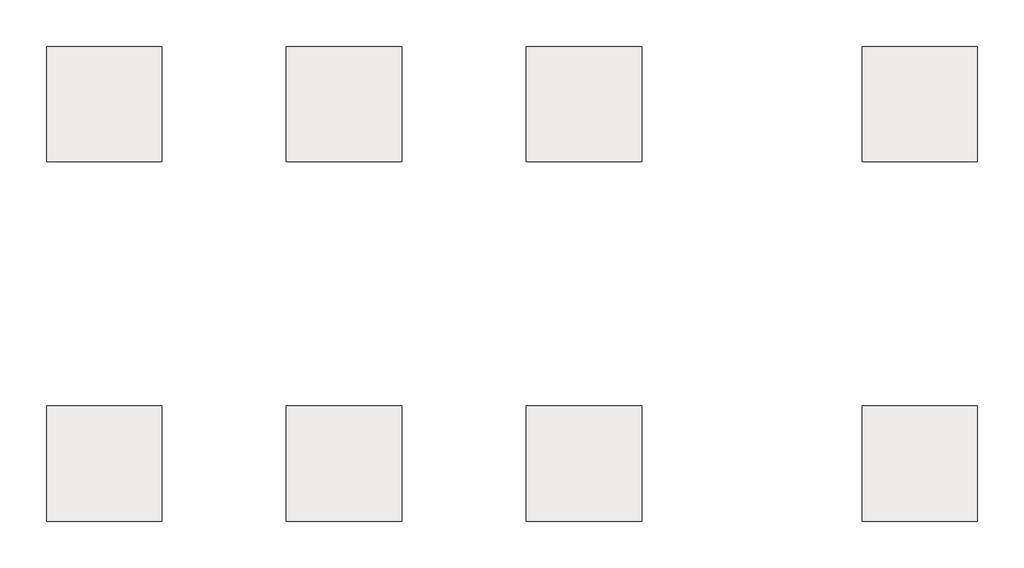
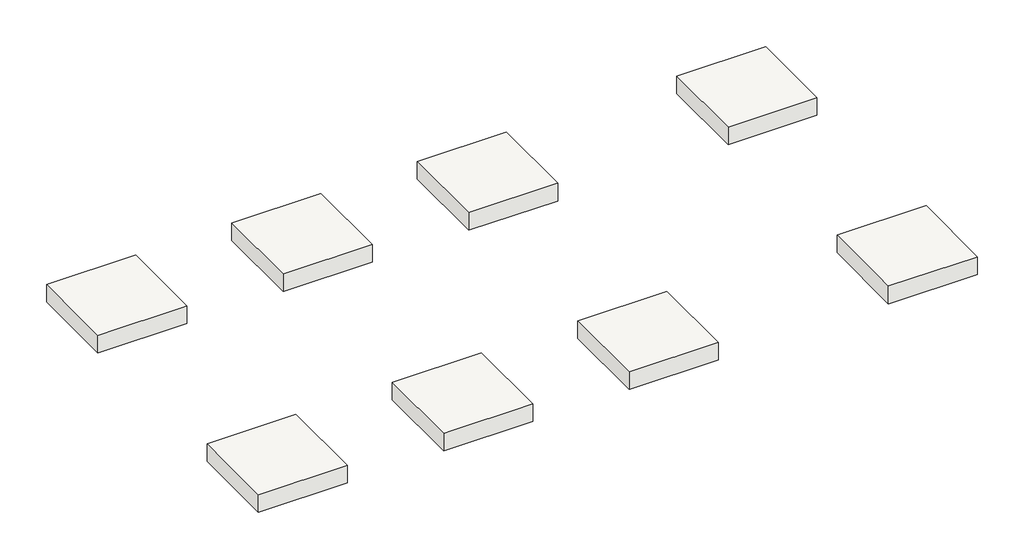
# Not in any storey: 8 slabs.
"""IFC4 building model written with IfcOpenShell, lengths in millimetres."""

import ifcopenshell
import ifcopenshell.guid

model = None  # the IFC model being written
_history = None  # IfcOwnerHistory: only IFC2X3 demands one
_inside = {}  # id of a spatial element -> (the spatial element, [elements in it])
_under = {}  # id of a project, library or spatial element -> (it, [spatial elements below it])
_declared = {}  # id of a project -> (the project, [libraries it declares])
_typed = {}  # id of a type object -> (the type object, [elements of that type])
_made_of = {}  # id of a material, layer set ... -> (it, [elements and type objects made of it])


def new_model(schema):
    """Start an empty IFC model of exactly this schema.

    Asked for "IFC4X3", IfcOpenShell would pick the latest addendum, in which some entities
    have other attributes; the version numbers below select the first issue.
    IFC2X3 requires an IfcOwnerHistory on every rooted entity: one is made here for all.
    """
    global model, _history
    if schema == "IFC4X3":
        model = ifcopenshell.file(schema_version=(4, 3, 0, 0))
    else:
        model = ifcopenshell.file(schema=schema)
    _inside.clear()
    _under.clear()
    _declared.clear()
    _typed.clear()
    _made_of.clear()
    _history = None
    if model.schema == "IFC2X3":
        org = make("IfcOrganization", Name="unknown")
        user = make(
            "IfcPersonAndOrganization",
            ThePerson=make("IfcPerson", FamilyName="unknown"),
            TheOrganization=org,
        )
        app = make(
            "IfcApplication",
            ApplicationDeveloper=org,
            Version="unknown",
            ApplicationFullName="unknown",
            ApplicationIdentifier="unknown",
        )
        _history = make(
            "IfcOwnerHistory",
            OwningUser=user,
            OwningApplication=app,
            ChangeAction="ADDED",
            CreationDate=0,
        )
    return model


def make(cls, **values):
    """One entity of the class cls with the attributes given. An attribute that is None is left unset."""
    return model.create_entity(
        cls, **{name: value for name, value in values.items() if value is not None}
    )


def rooted(cls, **values):
    """An entity with a GlobalId (a new one), such as an element, a storey or a relation."""
    return make(cls, GlobalId=ifcopenshell.guid.new(), OwnerHistory=_history, **values)


def si_unit(unit_type, name, prefix=None):
    """IfcSIUnit, for example si_unit("LENGTHUNIT", "METRE", prefix="MILLI")."""
    return make("IfcSIUnit", UnitType=unit_type, Prefix=prefix, Name=name)


def assignment(units):
    """IfcUnitAssignment: the units of a project."""
    return None if units is None else make("IfcUnitAssignment", Units=units)


def point(xyz):
    """IfcCartesianPoint."""
    return None if xyz is None else make("IfcCartesianPoint", Coordinates=xyz)


def direction(xyz):
    """IfcDirection."""
    return None if xyz is None else make("IfcDirection", DirectionRatios=xyz)


def frame(location, z_axis=None, x_axis=None):
    """IfcAxis2Placement3D, a coordinate frame: its origin and axes. An axis left out is left unset."""
    return make(
        "IfcAxis2Placement3D",
        Location=point(location),
        Axis=direction(z_axis),
        RefDirection=direction(x_axis),
    )


def origin():
    """The frame at (0, 0, 0) with its axes left unset."""
    return frame((0.0, 0.0, 0.0))


def place(relative_to, where):
    """IfcLocalPlacement: puts the frame where relative to a parent placement (None: the world)."""
    return make(
        "IfcLocalPlacement", PlacementRelTo=relative_to, RelativePlacement=where
    )


def context(
    kind, dimensions, precision=None, world=None, true_north=None, identifier=None
):
    """IfcGeometricRepresentationContext, for example the 3D "Model" context."""
    return make(
        "IfcGeometricRepresentationContext",
        ContextIdentifier=identifier,
        ContextType=kind,
        CoordinateSpaceDimension=dimensions,
        Precision=precision,
        WorldCoordinateSystem=world,
        TrueNorth=true_north,
    )


def project(units=None, contexts=None):
    """IfcProject with its units and contexts."""
    return rooted(
        "IfcProject",
        Name="project",
        RepresentationContexts=contexts,
        UnitsInContext=assignment(units),
    )


def spatial(cls, under=None, at=None, **own):
    """A site, building, storey or space (cls), placed at a placement, below another one or the project."""
    s = rooted(cls, ObjectPlacement=at, **own)
    if under is not None:
        _under.setdefault(under.id(), (under, []))[1].append(s)
    return s


def polyline(points):
    """IfcPolyline through the points."""
    return make("IfcPolyline", Points=[point(p) for p in points])


def outline(outer, holes=None, kind="AREA"):
    """IfcArbitraryClosedProfileDef: a profile drawn as a closed curve; with holes, ...WithVoids."""
    if holes is None:
        return make("IfcArbitraryClosedProfileDef", ProfileType=kind, OuterCurve=outer)
    return make(
        "IfcArbitraryProfileDefWithVoids",
        ProfileType=kind,
        OuterCurve=outer,
        InnerCurves=holes,
    )


def extrude(swept, where, along, depth):
    """IfcExtrudedAreaSolid: the profile swept, set in the frame where, extruded along a direction by depth."""
    return make(
        "IfcExtrudedAreaSolid",
        SweptArea=swept,
        Position=where,
        ExtrudedDirection=direction(along),
        Depth=depth,
    )


def shape(context_of_items, identifier, shape_type, items):
    """IfcShapeRepresentation: the items that make up one representation, for example the "Body"."""
    return make(
        "IfcShapeRepresentation",
        ContextOfItems=context_of_items,
        RepresentationIdentifier=identifier,
        RepresentationType=shape_type,
        Items=items,
    )


def source(mapping_origin, context_of_items, identifier, shape_type, items):
    """IfcRepresentationMap: a shape defined once, which mapped items show again and again."""
    return make(
        "IfcRepresentationMap",
        MappingOrigin=mapping_origin,
        MappedRepresentation=shape(context_of_items, identifier, shape_type, items),
    )


def transform(
    local_origin,
    x_axis=None,
    y_axis=None,
    z_axis=None,
    scale=None,
    scale2=None,
    scale3=None,
    uniform=True,
):
    """IfcCartesianTransformationOperator3D, or its non-uniform kind. x_axis, y_axis, z_axis: its Axis1, 2, 3."""
    if uniform:
        return make(
            "IfcCartesianTransformationOperator3D",
            Axis1=direction(x_axis),
            Axis2=direction(y_axis),
            LocalOrigin=point(local_origin),
            Scale=scale,
            Axis3=direction(z_axis),
        )
    return make(
        "IfcCartesianTransformationOperator3DnonUniform",
        Axis1=direction(x_axis),
        Axis2=direction(y_axis),
        LocalOrigin=point(local_origin),
        Scale=scale,
        Axis3=direction(z_axis),
        Scale2=scale2,
        Scale3=scale3,
    )


def mapped(mapping_source, mapping_target):
    """IfcMappedItem: shows the shape of a source again, moved by a transform."""
    return make(
        "IfcMappedItem", MappingSource=mapping_source, MappingTarget=mapping_target
    )


def made_of(thing, what):
    """Note that an element or type object is made of a material, layer set ...; save() writes the relation."""
    if what is not None:
        _made_of.setdefault(what.id(), (what, []))[1].append(thing)
    return thing


def element(
    cls,
    number,
    at=None,
    inside=None,
    cuts=None,
    type_object=None,
    material=None,
    context=None,
    identifier="Body",
    shape_type=None,
    held_by="IfcProductDefinitionShape",
    body=None,
    shapes=None,
    **own,
):
    """One element of the class cls, such as IfcWall. Its Tag is "e" and its number.

    at: its placement. inside: the storey or other place that contains it. cuts: it is an
    opening in that element (IfcRelVoidsElement). A single representation is given by context,
    identifier, shape_type and body (its items); several are given by shapes. held_by: the class
    of the entity that holds the representations. save() writes the other relations.
    """
    e = rooted(cls, Tag="e%d" % number, ObjectPlacement=at, **own)
    if body is not None:
        shapes = [shape(context, identifier, shape_type, body)]
    if shapes is not None:
        e.Representation = make(held_by, Representations=shapes)
    if inside is not None:
        _inside.setdefault(inside.id(), (inside, []))[1].append(e)
    if cuts is not None:
        rooted(
            "IfcRelVoidsElement", RelatingBuildingElement=cuts, RelatedOpeningElement=e
        )
    if type_object is not None:
        _typed.setdefault(type_object.id(), (type_object, []))[1].append(e)
    return made_of(e, material)


def aggregate(whole, parts):
    """IfcRelAggregates: a whole, such as a stair, and the parts it consists of."""
    return rooted("IfcRelAggregates", RelatingObject=whole, RelatedObjects=parts)


def save(model, path):
    """Write the relations noted so far, then the file.

    IfcRelAggregates (storeys below a building ...), IfcRelContainedInSpatialStructure (elements
    in a storey), IfcRelDefinesByType, IfcRelAssociatesMaterial and IfcRelDeclares: one each for
    every whole, place, type object, material and project.
    """
    for whole, parts in _under.values():
        aggregate(whole, parts)
    for where, things in _inside.values():
        rooted(
            "IfcRelContainedInSpatialStructure",
            RelatedElements=things,
            RelatingStructure=where,
        )
    for kind, things in _typed.values():
        rooted("IfcRelDefinesByType", RelatedObjects=things, RelatingType=kind)
    for what, things in _made_of.values():
        rooted("IfcRelAssociatesMaterial", RelatedObjects=things, RelatingMaterial=what)
    for by, libraries in _declared.values():
        rooted("IfcRelDeclares", RelatingContext=by, RelatedDefinitions=libraries)
    model.write(path)


def ft211_footing_rectangular_r0_ft211_footing_rectangular_5fe39465(model_context):
    return source(origin(), model_context, "Body", "SweptSolid", [
        extrude(outline(polyline([(1200.0, 1200.0), (1200.0, -1200.0), (-1200.0, -1200.0), (-1200.0, 1200.0), (1200.0, 1200.0)])), frame((0.0, 0.0, -500.0), z_axis=(0.0, 0.0, 1.0), x_axis=(1.0, 0.0, 0.0)), (0.0, 0.0, 1.0), 500.0),
    ])


model = new_model("IFC4")

# Units and contexts
model_context = context("Model", 3, world=origin())
ifc_project = project(units=[si_unit("LENGTHUNIT", "METRE", prefix="MILLI")], contexts=[model_context])

# Site, building
site = spatial("IfcSite", under=ifc_project)
building = spatial("IfcBuilding", under=site)

# Slabs
placement = place(None, origin())
element("IfcSlab", 1, ObjectType="FT211-Footing-Rectangular_R0 : FT211_Footing-Rectangular_2400x2400x500_F1", at=placement, inside=building, context=model_context, shape_type="SweptSolid", body=[
    extrude(outline(polyline([(11200.0, 22199.5208589), (11200.0, 19799.5208589), (8800.0, 19799.5208589), (8800.0, 22199.5208589), (11200.0, 22199.5208589)])), frame((0.0, 0.0, -1800.0), z_axis=(0.0, 0.0, 1.0), x_axis=(1.0, 0.0, 0.0)), (0.0, 0.0, 1.0), 500.0),
])
element("IfcSlab", 2, ObjectType="FT211-Footing-Rectangular_R0 : FT211_Footing-Rectangular_2400x2400x500_F1", at=placement, inside=building, context=model_context, shape_type="SweptSolid", body=[
    extrude(outline(polyline([(6200.0, 22199.5208589), (6200.0, 19799.5208589), (3800.0, 19799.5208589), (3800.0, 22199.5208589), (6200.0, 22199.5208589)])), frame((0.0, 0.0, -1800.0), z_axis=(0.0, 0.0, 1.0), x_axis=(1.0, 0.0, 0.0)), (0.0, 0.0, 1.0), 500.0),
])
element("IfcSlab", 3, ObjectType="FT211-Footing-Rectangular_R0 : FT211_Footing-Rectangular_2400x2400x500_F1", at=placement, inside=building, context=model_context, shape_type="SweptSolid", body=[
    extrude(outline(polyline([(1200.0, 22199.5208589), (1200.0, 19799.5208589), (-1200.0, 19799.5208589), (-1200.0, 22199.5208589), (1200.0, 22199.5208589)])), frame((0.0, 0.0, -1800.0), z_axis=(0.0, 0.0, 1.0), x_axis=(1.0, 0.0, 0.0)), (0.0, 0.0, 1.0), 500.0),
])
element("IfcSlab", 4, ObjectType="FT211-Footing-Rectangular_R0 : FT211_Footing-Rectangular_2400x2400x500_F1", at=placement, inside=building, context=model_context, shape_type="SweptSolid", body=[
    extrude(outline(polyline([(1200.0, 14699.5208589), (1200.0, 12299.5208589), (-1200.0, 12299.5208589), (-1200.0, 14699.5208589), (1200.0, 14699.5208589)])), frame((0.0, 0.0, -1800.0), z_axis=(0.0, 0.0, 1.0), x_axis=(1.0, 0.0, 0.0)), (0.0, 0.0, 1.0), 500.0),
])
element("IfcSlab", 5, ObjectType="FT211-Footing-Rectangular_R0 : FT211_Footing-Rectangular_2400x2400x500_F1", at=placement, inside=building, context=model_context, shape_type="SweptSolid", body=[
    extrude(outline(polyline([(18200.0, 22199.5208589), (18200.0, 19799.5208589), (15800.0, 19799.5208589), (15800.0, 22199.5208589), (18200.0, 22199.5208589)])), frame((0.0, 0.0, -1800.0), z_axis=(0.0, 0.0, 1.0), x_axis=(1.0, 0.0, 0.0)), (0.0, 0.0, 1.0), 500.0),
])
ft211_footing_rectangular_r0_ft211_footing_rectangular_shape = ft211_footing_rectangular_r0_ft211_footing_rectangular_5fe39465(model_context)
element("IfcSlab", 6, ObjectType="FT211-Footing-Rectangular_R0 : FT211_Footing-Rectangular_2400x2400x500_F1", at=placement, inside=building, context=model_context, shape_type="MappedRepresentation", body=[
    mapped(ft211_footing_rectangular_r0_ft211_footing_rectangular_shape, transform((5000.0, 13499.5208589, -1300.0), x_axis=(1.0, 0.0, 0.0), y_axis=(0.0, 1.0, 0.0), z_axis=(0.0, 0.0, 1.0))),
])
element("IfcSlab", 7, ObjectType="FT211-Footing-Rectangular_R0 : FT211_Footing-Rectangular_2400x2400x500_F1", at=placement, inside=building, context=model_context, shape_type="MappedRepresentation", body=[
    mapped(ft211_footing_rectangular_r0_ft211_footing_rectangular_shape, transform((10000.0, 13499.5208589, -1300.0), x_axis=(1.0, 0.0, 0.0), y_axis=(0.0, 1.0, 0.0), z_axis=(0.0, 0.0, 1.0))),
])
element("IfcSlab", 8, ObjectType="FT211-Footing-Rectangular_R0 : FT211_Footing-Rectangular_2400x2400x500_F1", at=placement, inside=building, context=model_context, shape_type="MappedRepresentation", body=[
    mapped(ft211_footing_rectangular_r0_ft211_footing_rectangular_shape, transform((17000.0, 13499.5208589, -1300.0), x_axis=(1.0, 0.0, 0.0), y_axis=(0.0, 1.0, 0.0), z_axis=(0.0, 0.0, 1.0))),
])

save(model, "model.ifc")

# Revit data of these elements
# Project information
#   Building Name = "MAIN GATE SECURITY BUILDING"
#   Project Status = "Project Status"
#   Client Name = "현대엔지니어링"
#   Project Address = "서울시 종로구 율곡로 75(계동)"
#   Project Name = "Therma Visayas Energy Project"
#   Project Number = "-"
# Grids (mm)
#   "A": line (0, 24502.793) -> (0, 11308.625)
#   "B": line (5000, 24502.793) -> (5000, 11308.625)
#   "C": line (10000, 24502.793) -> (10000, 11308.625)
#   "1": line (-3860.098, 13499.521) -> (12441.468, 13499.521)
#   "2": line (-3860.098, 20999.521) -> (12441.468, 20999.521)
# Type "FT211-Footing-Rectangular_R0 : FT211_Footing-Rectangular_2400x2400x500_F1"
#   Top bar = "D25@300"
#   Description = "UG Shallow Foundation"
#   Bottom bar = "D20@300"
#   Width = 2400 mm
#   Length = 2400 mm
#   Foundation Thickness = 500 mm
#   Structural Material [instance default] = A03AC032-00007_Structural Concrete_Type1_25MPa-30Mpa
#   Assembly Code = ""
# Elements 1, 2, 3, 4, 6, 7 (IfcSlab, "FT211-Footing-Rectangular_R0 : FT211_Footing-Rectangular_2400x2400x500_F1")
#   Comments = ""
#   Mark = "F1"
#   F01) Building Name = "Main Gate House"
#   F11) Project Building Tag_Type-1 = "Common"
#   F12) Project Building Tag_Type-2 = "Common"
#   F13) Project Facility Code = "Facility Code"
#   F21) Structural Type = "Concrete"
#   F31) Standard Building Code = "IBC"
#   F41) Discipline = "AR"
#   F51) Plan Start Date-Engineering = "2015-01-01"
#   F52) Plan Finish Date-Engineering = "2015-12-31"
#   F53) Duration = "365"
#   F54) Actual Start Date-Engineering = "2015-01-01"
#   F55) Actual Finish Date-Engineering = "2015-12-31"
#   F61) Plan Start Date-Construction = "2016-08-19"
#   F62) Plan Finish Date-Construction = "2017-01-31"
#   F64) Actual Start Date-Construction = "2016-08-19"
#   F63) Duration = "202"
#   F65) Actual Finish Date-Construction = "2017-01-31"
#   F91) Plant Type = "CFPP"
#   F92) KKS Structures, Building = "UYF"
#   P01) Project Name = "TVEP"
#   P02) Project Configuration = "CFB Boiler x 2(Foster Wheeler) + STG x 2(Alstom, 150MW)"
#   P03) Project Abbreviation = "TVEP"
#   P04) Project Code = "BEPH1402"
#   P05) Project Stage = "In operation"
#   P06) Project Location = "Sito Looc, Barangay Bato, Toledo City in Philippines"
#   P07) Project Owner = "Therma Visayas, Inc."
#   P08) Project O.E = "Flour"
#   P09) Project Schedule = "ITB Issueing Date : 2013.07.30\r\nSite Survey : 2013.08.19-20\r\nBid Closing Date : 2013.11.29\r\nPreferred Bidder Notice 접수 : 2014.04.27\r\nTarget award date : 2014 05\r\nLOA 접수 : 2014.05.21\r\nSigning Ceremony : 2014.05.30"
#   P10) Basic Wind Speed = "55.6 m/s"
#   P11) Seismic = "NSCP 2010, Zone 4 (PGA : 0.4g)"
#   P12) Soil = "Sc"
#   P13) Soil Capacity = "100kN/m2"
#   P14) Pile Capacity = "PHC(D400) : 1200kN"
#   W00) Work Master Code = "A03AC032-00007"
#   W01) Work Master_Lv1 = "Concrete Work"
#   W02) Work Master_Lv2 = "Substructure Work"
#   W03) Work Master_Spec.1 = "Cement Type-1"
#   W04) Work Master_Spec.2 = "25MPa < F'c (Cylinder Strength) ≤ 30MPa"
#   W11) Activity ID = "C02AGB010"
#   W12) Activity Name = "Main Gate Security Building - Building Foundation"
#   W13) Plan Start Date = "2016-08-19"
#   W14) Plan Finish Date = "2016-09-22"
#   W15) Duration = "26"
#   W16) Actual Start Date = "2016-08-19"
#   W17) Actual Finish Date = "2016-09-22"
#   R02) Unit Price = 0
#   Structural Material = A03AC032-00007_Structural Concrete_Type1_25MPa-30Mpa
#   Phase Created = New Construction
#   Materials on its faces: "A03AC032-00007_Structural Concrete_Type1_25MPa-30Mpa"
# Elements 5, 8 (IfcSlab, "FT211-Footing-Rectangular_R0 : FT211_Footing-Rectangular_2400x2400x500_F1")
#   Comments = ""
#   F01) Building Name = "Main Gate House"
#   F11) Project Building Tag_Type-1 = "Common"
#   F12) Project Building Tag_Type-2 = "Common"
#   F13) Project Facility Code = "Facility Code"
#   F21) Structural Type = "Concrete"
#   F31) Standard Building Code = "IBC"
#   F41) Discipline = "AR"
#   F51) Plan Start Date-Engineering = "2015-01-01"
#   F52) Plan Finish Date-Engineering = "2015-12-31"
#   F53) Duration = "365"
#   F54) Actual Start Date-Engineering = "2015-01-01"
#   F55) Actual Finish Date-Engineering = "2015-12-31"
#   F61) Plan Start Date-Construction = "2016-08-19"
#   F62) Plan Finish Date-Construction = "2017-01-31"
#   F64) Actual Start Date-Construction = "2016-08-19"
#   F63) Duration = "202"
#   F65) Actual Finish Date-Construction = "2017-01-31"
#   F91) Plant Type = "CFPP"
#   F92) KKS Structures, Building = "UYF"
#   P01) Project Name = "TVEP"
#   P02) Project Configuration = "CFB Boiler x 2(Foster Wheeler) + STG x 2(Alstom, 150MW)"
#   P03) Project Abbreviation = "TVEP"
#   P04) Project Code = "BEPH1402"
#   P05) Project Stage = "In operation"
#   P06) Project Location = "Sito Looc, Barangay Bato, Toledo City in Philippines"
#   P07) Project Owner = "Therma Visayas, Inc."
#   P08) Project O.E = "Flour"
#   P09) Project Schedule = "ITB Issueing Date : 2013.07.30\r\nSite Survey : 2013.08.19-20\r\nBid Closing Date : 2013.11.29\r\nPreferred Bidder Notice 접수 : 2014.04.27\r\nTarget award date : 2014 05\r\nLOA 접수 : 2014.05.21\r\nSigning Ceremony : 2014.05.30"
#   P10) Basic Wind Speed = "55.6 m/s"
#   P11) Seismic = "NSCP 2010, Zone 4 (PGA : 0.4g)"
#   P12) Soil = "Sc"
#   P13) Soil Capacity = "100kN/m2"
#   P14) Pile Capacity = "PHC(D400) : 1200kN"
#   W00) Work Master Code = "A03AC032-00007"
#   W01) Work Master_Lv1 = "Concrete Work"
#   W02) Work Master_Lv2 = "Substructure Work"
#   W03) Work Master_Spec.1 = "Cement Type-1"
#   W04) Work Master_Spec.2 = "25MPa < F'c (Cylinder Strength) ≤ 30MPa"
#   W11) Activity ID = "C02AGB010"
#   W12) Activity Name = "Main Gate Security Building - Building Foundation"
#   W13) Plan Start Date = "2016-08-19"
#   W14) Plan Finish Date = "2016-09-22"
#   W15) Duration = "26"
#   W16) Actual Start Date = "2016-08-19"
#   W17) Actual Finish Date = "2016-09-22"
#   R02) Unit Price = 0
#   Structural Material = A03AC032-00007_Structural Concrete_Type1_25MPa-30Mpa
#   Phase Created = New Construction
#   Materials on its faces: "A03AC032-00007_Structural Concrete_Type1_25MPa-30Mpa"
# Materials
#   "A03AC032-00007_Structural Concrete_Type1_25MPa-30Mpa": class "Concrete", colour RGB 176 176 176, transparency 0, Keynote = "09910.A1", Description = "Reinf. Conc.", W00) Work Master Code = "A03AC032-00007", W01) Work Master_Lv1 = "Concrete Work", W02) Work Master_Lv2 = "Substructure Work", W03) Work Master_Spec.1 = "Structural Concrete", W04) Work Master_Spec.2 = "Cement Type-1", W05) Work Master_Spec.3 = "25MPa < F'c (Cylinder Strength) ≤ 30MPa", Cost = 0
